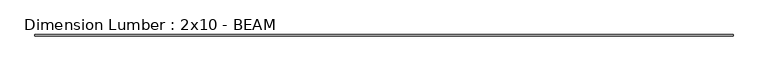
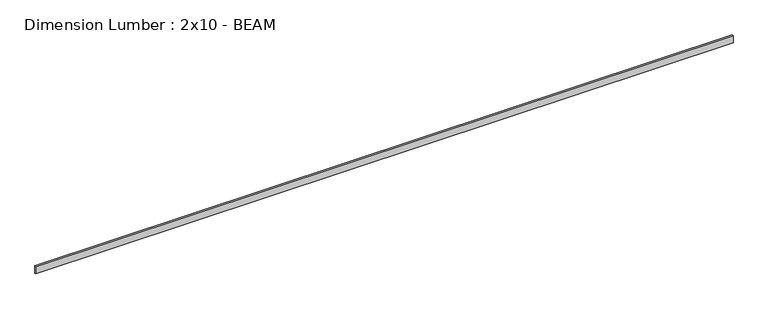
"""IFC4 building model written with IfcOpenShell, lengths in millimetres: beam geometry, Dimension Lumber : 2x10 - BEAM."""

from ifc_helpers import new_model, si_unit, frame, origin, place, context, project, spatial, polyline, outline, extrude, source, transform, mapped, element, save


def dimension_lumber_2x10_beam_07621911(model_context):
    return source(origin(), model_context, "Body", "SweptSolid", [
        extrude(outline(polyline([(10509.25, 19.05), (10509.25, -19.05), (-10768.0125, -19.05), (-10768.0125, 19.05), (10509.25, 19.05)])), frame((0.0, 0.0, -117.475), z_axis=(0.0, 0.0, 1.0), x_axis=(1.0, 0.0, 0.0)), (0.0, 0.0, 1.0), 234.95),
    ])


if __name__ == "__main__":
    model = new_model("IFC4")
    model_context = context("Model", 3, world=origin())
    ifc_project = project(units=[si_unit("LENGTHUNIT", "METRE", prefix="MILLI")], contexts=[model_context])
    site = spatial("IfcSite", under=ifc_project)
    building = spatial("IfcBuilding", under=site)
    placement = place(None, origin())
    dimension_lumber_2x10_beam_shape = dimension_lumber_2x10_beam_07621911(model_context)
    element("IfcBeam", 1, ObjectType="Dimension Lumber : 2x10 - BEAM", at=placement, inside=building, context=model_context, shape_type="MappedRepresentation", body=[
        mapped(dimension_lumber_2x10_beam_shape, transform((0.0, 0.0, 0.0), x_axis=(1.0, 0.0, 0.0), y_axis=(0.0, 1.0, 0.0), z_axis=(0.0, 0.0, 1.0))),
    ])
    save(model, "model.ifc")

# Revit data of these elements
# Type "Dimension Lumber : 2x10 - BEAM"
#   Assembly Code = "B10"
#   A = 0.0755556 SF
#   Length [instance default] = 5' - 0"
#   b = 0' - 1 1/2"
#   d = 0' - 9 1/4"
#   Structural Material = (3) SISTERED 2X10s AT BEAM
# Element 1 (IfcBeam, "Dimension Lumber : 2x10 - BEAM")
#   Materials on its faces: "(3) SISTERED 2X10s AT BEAM"
# Materials
#   "(3) SISTERED 2X10s AT BEAM": class "Wood", colour RGB 234 198 147, transparency 0, Description = "Pinus Echinata", Cost = 0
